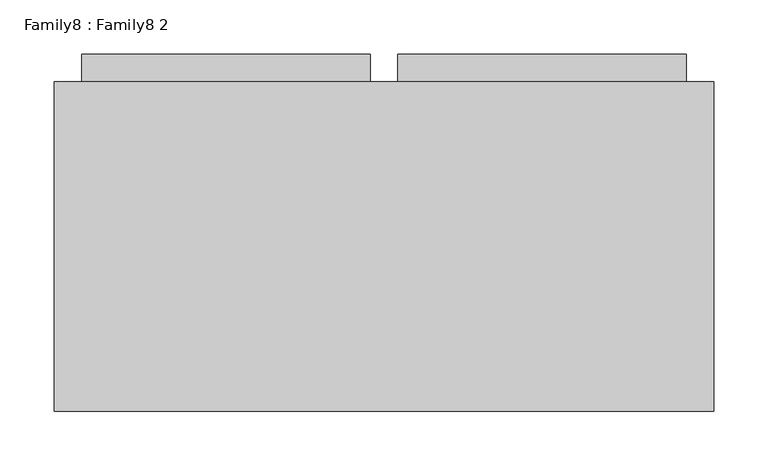
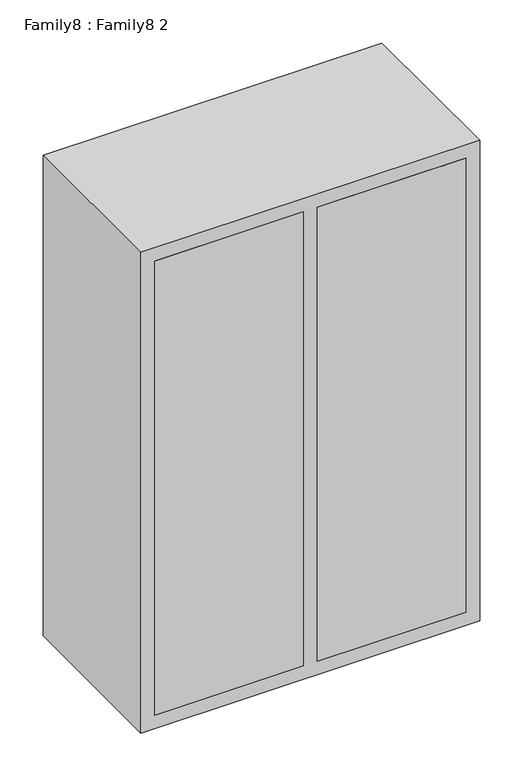
"""IFC4 building model written with IfcOpenShell, lengths in millimetres: proxy geometry, Family8 : Family8 2."""

from ifc_helpers import new_model, si_unit, frame, origin, place, context, project, spatial, polyline, outline, extrude, source, transform, mapped, element, save


def family8_family8_2_f16280a4(model_context):
    return source(origin(), model_context, "Body", "SweptSolid", [
        extrude(outline(polyline([(12.7, 381.0), (279.4, 381.0), (279.4, 50.8), (12.7, 50.8), (12.7, 381.0)])), frame((0.0, 0.0, 1499.5130448), z_axis=(0.0, 0.0, 1.0), x_axis=(1.0, 0.0, 0.0)), (0.0, 0.0, 1.0), 863.6),
        extrude(outline(polyline([(-279.4, 381.0), (-12.7, 381.0), (-12.7, 50.8), (-279.4, 50.8), (-279.4, 381.0)])), frame((0.0, 0.0, 1499.5130448), z_axis=(0.0, 0.0, 1.0), x_axis=(1.0, 0.0, 0.0)), (0.0, 0.0, 1.0), 863.6),
        extrude(outline(polyline([(-304.8, 355.6), (304.8, 355.6), (304.8, 50.8), (-304.8, 50.8), (-304.8, 355.6)])), frame((0.0, 0.0, 1474.1130448), z_axis=(0.0, 0.0, 1.0), x_axis=(1.0, 0.0, 0.0)), (0.0, 0.0, 1.0), 914.4),
    ])


if __name__ == "__main__":
    model = new_model("IFC4")
    model_context = context("Model", 3, world=origin())
    ifc_project = project(units=[si_unit("LENGTHUNIT", "METRE", prefix="MILLI")], contexts=[model_context])
    site = spatial("IfcSite", under=ifc_project)
    building = spatial("IfcBuilding", under=site)
    placement = place(None, origin())
    family8_family8_2_shape = family8_family8_2_f16280a4(model_context)
    element("IfcBuildingElementProxy", 1, Name="Family8 : Family8 2", ObjectType="Family8 : Family8 2", at=placement, inside=building, context=model_context, shape_type="MappedRepresentation", body=[
        mapped(family8_family8_2_shape, transform((0.0, 0.0, 0.0), x_axis=(1.0, 0.0, 0.0), y_axis=(0.0, 1.0, 0.0), z_axis=(0.0, 0.0, 1.0))),
    ])
    save(model, "model.ifc")

# Revit data of these elements
# Type "Family8 : Family8 2"
#   total width = 2' - 0"
#   drawer depth = 1' - 1"
#   cabinet depth = 1' - 0"
#   Default Elevation = 0
